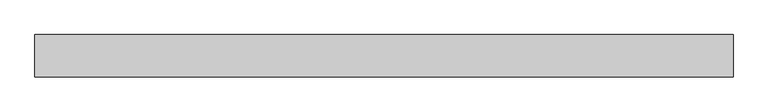
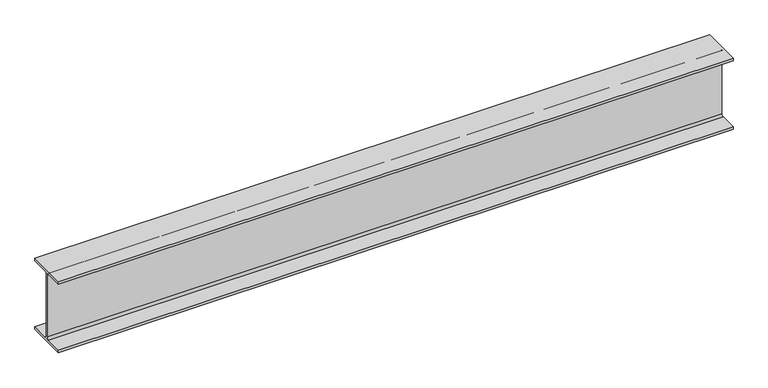
"""IFC4 building model written with IfcOpenShell, lengths in millimetres: beam geometry, Steel Beam_H-KSD3502 : H_SB_ASB_H-194x150x6x9."""

from ifc_helpers import new_model, si_unit, point, frame, frame_2d, origin, place, context, project, spatial, polyline, circle_curve, trimmed, segment, composite_curve, outline, extrude, source, transform, mapped, element, save


def beam_157ca0d3(model_context):
    return source(origin(), model_context, "Body", "SweptSolid", [
        extrude(outline(composite_curve([segment(polyline([(82.5, -141.5), (82.5, -151.7), (-82.5, -151.7), (-82.5, -141.5), (-11.9, -141.5)]), True, "CONTINUOUS"), segment(trimmed(circle_curve(frame_2d((-11.9, -132.6)), 8.9), [point((-11.9, -141.5))], [point((-3.0, -132.6))], True, "CARTESIAN"), True, "CONTINUOUS"), segment(polyline([(-3.0, -132.6), (-3.0, 132.6)]), True, "CONTINUOUS"), segment(trimmed(circle_curve(frame_2d((-11.9, 132.6)), 8.9), [point((-3.0, 132.6))], [point((-11.9, 141.5))], True, "CARTESIAN"), True, "CONTINUOUS"), segment(polyline([(-11.9, 141.5), (-82.5, 141.5), (-82.5, 151.7), (82.5, 151.7), (82.5, 141.5), (11.9, 141.5)]), True, "CONTINUOUS"), segment(trimmed(circle_curve(frame_2d((11.9, 132.6)), 8.9), [point((11.9, 141.5))], [point((3.0, 132.6))], True, "CARTESIAN"), True, "CONTINUOUS"), segment(polyline([(3.0, 132.6), (3.0, -132.6)]), True, "CONTINUOUS"), segment(trimmed(circle_curve(frame_2d((11.9, -132.6)), 8.9), [point((3.0, -132.6))], [point((11.9, -141.5))], True, "CARTESIAN"), True, "CONTINUOUS"), segment(polyline([(11.9, -141.5), (82.5, -141.5)]), True, "CONTINUOUS")], self_intersect=False)), frame((-1236.0559406, 0.0, 0.0), z_axis=(1.0, 0.0, 0.0), x_axis=(0.0, 1.0, 0.0)), (0.0, 0.0, 1.0), 2729.2385396),
    ])


if __name__ == "__main__":
    model = new_model("IFC4")
    model_context = context("Model", 3, world=origin())
    ifc_project = project(units=[si_unit("LENGTHUNIT", "METRE", prefix="MILLI")], contexts=[model_context])
    site = spatial("IfcSite", under=ifc_project)
    building = spatial("IfcBuilding", under=site)
    placement = place(None, origin())
    beam_shape = beam_157ca0d3(model_context)
    element("IfcBeam", 1, ObjectType="Steel Beam_H-KSD3502 : H_SB_ASB_H-194x150x6x9", at=placement, inside=building, context=model_context, shape_type="MappedRepresentation", body=[
        mapped(beam_shape, transform((0.0, 0.0, 0.0), x_axis=(1.0, 0.0, 0.0), y_axis=(0.0, 1.0, 0.0), z_axis=(0.0, 0.0, 1.0))),
    ])
    save(model, "model.ifc")

# Revit data of these elements
# Type "Steel Beam_H-KSD3502 : H_SB_ASB_H-194x150x6x9"
#   Width = 15.0 cm
#   Web Thickness = 0.6 cm
#   Web Fillet = 1.3 cm
#   Warping Constant = 43316.0 cm⁶
#   Torsional Moment of Inertia = 8.622 cm⁴
#   Torsional Modulus = 1.0 cm³
#   Section Area = 39.01 cm²
#   Plastic Modulus weak axis = 104.0 cm³
#   Plastic Modulus strong axis = 309.0 cm³
#   Perimeter = 0.95 m²/m
#   Nominal Weight = 30.60 kgf/m
#   Moment of Inertia weak axis = 507.00 cm⁴
#   Moment of Inertia strong axis = 2690.00 cm⁴
#   Height = 19.4 cm
#   Flange Thickness = 0.9 cm
#   Elastic Modulus weak axis = 67.6 cm³
#   Elastic Modulus strong axis = 277.0 cm³
#   Centroid Vertical = 9.7 cm
#   Centroid Horizontal = 7.5 cm
#   Length [instance default] = 1.5240 m
#   Structural Material [instance default] = Steel, 45-345
#   Assembly Code = ""
# Element 1 (IfcBeam, "Steel Beam_H-KSD3502 : H_SB_ASB_H-194x150x6x9")
#   Structural Material = none
# Materials
#   "Steel, 45-345": class "Metal", colour RGB 189 187 185, transparency 0, Description = "Steel 345 MPa", Cost = 0
